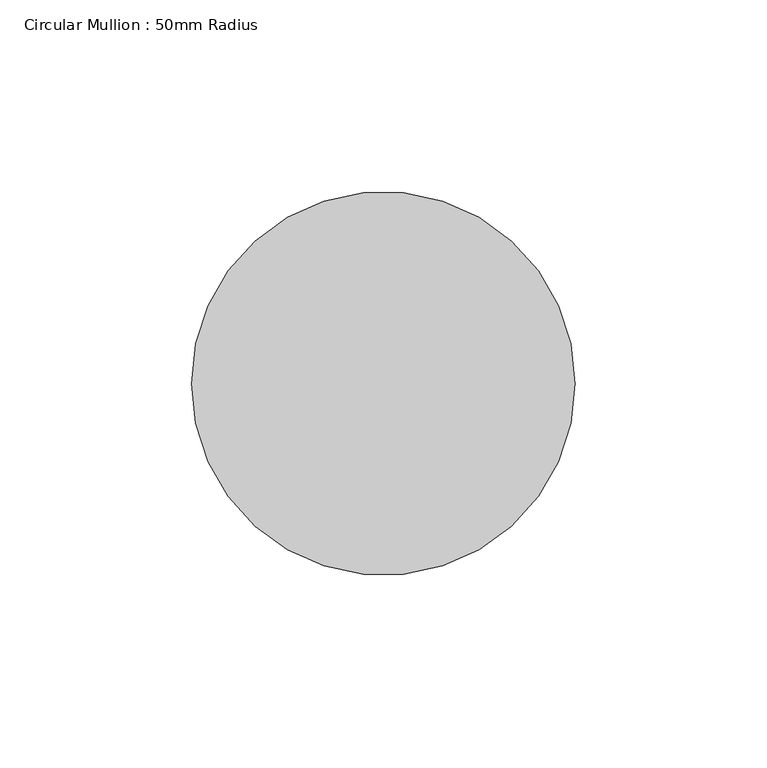
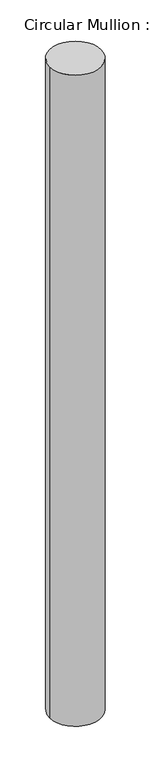
"""IFC4 building model written with IfcOpenShell, lengths in millimetres: member geometry, Circular Mullion : 50mm Radius."""

from ifc_helpers import new_model, si_unit, point, frame, origin, origin_2d, place, context, project, spatial, circle_curve, trimmed, segment, composite_curve, outline, extrude, source, transform, mapped, element, save


def circular_mullion_50mm_radius_b69e5350(model_context):
    return source(origin(), model_context, "Body", "SweptSolid", [
        extrude(outline(composite_curve([segment(trimmed(circle_curve(origin_2d(), 50.0), [point((50.0, 0.0))], [point((-50.0, 0.0))], False, "CARTESIAN"), True, "CONTINUOUS"), segment(trimmed(circle_curve(origin_2d(), 50.0), [point((-50.0, 0.0))], [point((50.0, 0.0))], False, "CARTESIAN"), True, "CONTINUOUS")], self_intersect=False)), frame((0.0, 0.0, -1334.9847918), z_axis=(0.0, 0.0, 1.0), x_axis=(1.0, 0.0, 0.0)), (0.0, 0.0, 1.0), 1334.9847918),
    ])


if __name__ == "__main__":
    model = new_model("IFC4")
    model_context = context("Model", 3, world=origin())
    ifc_project = project(units=[si_unit("LENGTHUNIT", "METRE", prefix="MILLI")], contexts=[model_context])
    site = spatial("IfcSite", under=ifc_project)
    building = spatial("IfcBuilding", under=site)
    placement = place(None, origin())
    circular_mullion_50mm_radius_shape = circular_mullion_50mm_radius_b69e5350(model_context)
    element("IfcMember", 1, ObjectType="Circular Mullion : 50mm Radius", at=placement, inside=building, context=model_context, shape_type="MappedRepresentation", body=[
        mapped(circular_mullion_50mm_radius_shape, transform((0.0, 0.0, 0.0), x_axis=(1.0, 0.0, 0.0), y_axis=(0.0, 1.0, 0.0), z_axis=(0.0, 0.0, 1.0))),
    ])
    save(model, "model.ifc")

# Revit data of these elements
# Type "Circular Mullion : 50mm Radius"
#   built-in parameter 1007350 = 0.164042 (stored number, unit not read)
# Element 1 (IfcMember, "Circular Mullion : 50mm Radius")
#   Materials on its faces: "Aluminium"
# Materials
#   "Aluminium": class "Metal", colour RGB 247 247 247, transparency 0, Description = "Aluminium 6061", Cost = 0
